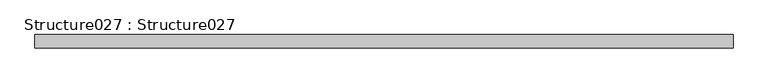
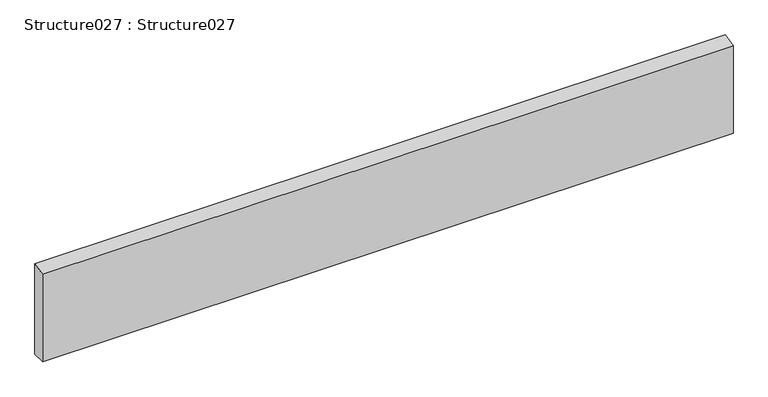
"""IFC4 building model written with IfcOpenShell, lengths in millimetres: proxy geometry, Structure027 : Structure027."""

from ifc_helpers import new_model, si_unit, frame, origin, place, context, project, spatial, polyline, outline, extrude, source, transform, mapped, element, save


def structure027_structure027_0c995fee(model_context):
    return source(origin(), model_context, "Body", "SweptSolid", [
        extrude(outline(polyline([(-4351.8279009, 43018.9246048), (-4351.8279009, 42741.596), (-4389.9279009, 42741.596), (-4389.9279009, 43009.3996048), (-4351.8279009, 43018.9246048)])), frame((12382.7678845, 0.0, 0.0), z_axis=(1.0, 0.0, 0.0), x_axis=(0.0, 1.0, 0.0)), (0.0, 0.0, 1.0), 2000.25),
    ])


if __name__ == "__main__":
    model = new_model("IFC4")
    model_context = context("Model", 3, world=origin())
    ifc_project = project(units=[si_unit("LENGTHUNIT", "METRE", prefix="MILLI")], contexts=[model_context])
    site = spatial("IfcSite", under=ifc_project)
    building = spatial("IfcBuilding", under=site)
    placement = place(None, origin())
    structure027_structure027_shape = structure027_structure027_0c995fee(model_context)
    element("IfcBuildingElementProxy", 1, Name="Structure027 : Structure027", ObjectType="Structure027 : Structure027", at=placement, inside=building, context=model_context, shape_type="MappedRepresentation", body=[
        mapped(structure027_structure027_shape, transform((0.0, 0.0, 0.0), x_axis=(1.0, 0.0, 0.0), y_axis=(0.0, 1.0, 0.0), z_axis=(0.0, 0.0, 1.0))),
    ])
    save(model, "model.ifc")

# Revit data of these elements
# Type "Structure027 : Structure027"
#   NameOverride = "Structure027"
# Element 1 (IfcBuildingElementProxy, "Structure027 : Structure027")
#   Materials on its faces: "2x BLOCKING AS NECESSARY"
# Materials
#   "2x BLOCKING AS NECESSARY": class "Unassigned", colour RGB 166 124 85, transparency 0, Cost = 0
